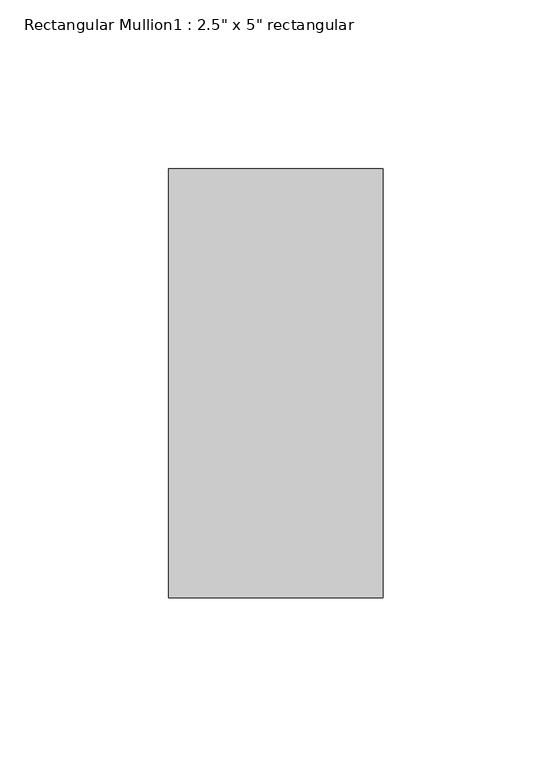
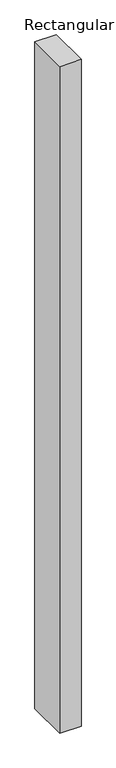
"""IFC4 building model written with IfcOpenShell, lengths in millimetres: member geometry."""

import ifcopenshell
import ifcopenshell.guid

model = None  # the IFC model being written
_history = None  # IfcOwnerHistory: only IFC2X3 demands one
_inside = {}  # id of a spatial element -> (the spatial element, [elements in it])
_under = {}  # id of a project, library or spatial element -> (it, [spatial elements below it])
_declared = {}  # id of a project -> (the project, [libraries it declares])
_typed = {}  # id of a type object -> (the type object, [elements of that type])
_made_of = {}  # id of a material, layer set ... -> (it, [elements and type objects made of it])


def new_model(schema):
    """Start an empty IFC model of exactly this schema.

    Asked for "IFC4X3", IfcOpenShell would pick the latest addendum, in which some entities
    have other attributes; the version numbers below select the first issue.
    IFC2X3 requires an IfcOwnerHistory on every rooted entity: one is made here for all.
    """
    global model, _history
    if schema == "IFC4X3":
        model = ifcopenshell.file(schema_version=(4, 3, 0, 0))
    else:
        model = ifcopenshell.file(schema=schema)
    _inside.clear()
    _under.clear()
    _declared.clear()
    _typed.clear()
    _made_of.clear()
    _history = None
    if model.schema == "IFC2X3":
        org = make("IfcOrganization", Name="unknown")
        user = make(
            "IfcPersonAndOrganization",
            ThePerson=make("IfcPerson", FamilyName="unknown"),
            TheOrganization=org,
        )
        app = make(
            "IfcApplication",
            ApplicationDeveloper=org,
            Version="unknown",
            ApplicationFullName="unknown",
            ApplicationIdentifier="unknown",
        )
        _history = make(
            "IfcOwnerHistory",
            OwningUser=user,
            OwningApplication=app,
            ChangeAction="ADDED",
            CreationDate=0,
        )
    return model


def make(cls, **values):
    """One entity of the class cls with the attributes given. An attribute that is None is left unset."""
    return model.create_entity(
        cls, **{name: value for name, value in values.items() if value is not None}
    )


def rooted(cls, **values):
    """An entity with a GlobalId (a new one), such as an element, a storey or a relation."""
    return make(cls, GlobalId=ifcopenshell.guid.new(), OwnerHistory=_history, **values)


def si_unit(unit_type, name, prefix=None):
    """IfcSIUnit, for example si_unit("LENGTHUNIT", "METRE", prefix="MILLI")."""
    return make("IfcSIUnit", UnitType=unit_type, Prefix=prefix, Name=name)


def assignment(units):
    """IfcUnitAssignment: the units of a project."""
    return None if units is None else make("IfcUnitAssignment", Units=units)


def point(xyz):
    """IfcCartesianPoint."""
    return None if xyz is None else make("IfcCartesianPoint", Coordinates=xyz)


def direction(xyz):
    """IfcDirection."""
    return None if xyz is None else make("IfcDirection", DirectionRatios=xyz)


def frame(location, z_axis=None, x_axis=None):
    """IfcAxis2Placement3D, a coordinate frame: its origin and axes. An axis left out is left unset."""
    return make(
        "IfcAxis2Placement3D",
        Location=point(location),
        Axis=direction(z_axis),
        RefDirection=direction(x_axis),
    )


def origin():
    """The frame at (0, 0, 0) with its axes left unset."""
    return frame((0.0, 0.0, 0.0))


def place(relative_to, where):
    """IfcLocalPlacement: puts the frame where relative to a parent placement (None: the world)."""
    return make(
        "IfcLocalPlacement", PlacementRelTo=relative_to, RelativePlacement=where
    )


def context(
    kind, dimensions, precision=None, world=None, true_north=None, identifier=None
):
    """IfcGeometricRepresentationContext, for example the 3D "Model" context."""
    return make(
        "IfcGeometricRepresentationContext",
        ContextIdentifier=identifier,
        ContextType=kind,
        CoordinateSpaceDimension=dimensions,
        Precision=precision,
        WorldCoordinateSystem=world,
        TrueNorth=true_north,
    )


def project(units=None, contexts=None):
    """IfcProject with its units and contexts."""
    return rooted(
        "IfcProject",
        Name="project",
        RepresentationContexts=contexts,
        UnitsInContext=assignment(units),
    )


def spatial(cls, under=None, at=None, **own):
    """A site, building, storey or space (cls), placed at a placement, below another one or the project."""
    s = rooted(cls, ObjectPlacement=at, **own)
    if under is not None:
        _under.setdefault(under.id(), (under, []))[1].append(s)
    return s


def polyline(points):
    """IfcPolyline through the points."""
    return make("IfcPolyline", Points=[point(p) for p in points])


def outline(outer, holes=None, kind="AREA"):
    """IfcArbitraryClosedProfileDef: a profile drawn as a closed curve; with holes, ...WithVoids."""
    if holes is None:
        return make("IfcArbitraryClosedProfileDef", ProfileType=kind, OuterCurve=outer)
    return make(
        "IfcArbitraryProfileDefWithVoids",
        ProfileType=kind,
        OuterCurve=outer,
        InnerCurves=holes,
    )


def extrude(swept, where, along, depth):
    """IfcExtrudedAreaSolid: the profile swept, set in the frame where, extruded along a direction by depth."""
    return make(
        "IfcExtrudedAreaSolid",
        SweptArea=swept,
        Position=where,
        ExtrudedDirection=direction(along),
        Depth=depth,
    )


def shape(context_of_items, identifier, shape_type, items):
    """IfcShapeRepresentation: the items that make up one representation, for example the "Body"."""
    return make(
        "IfcShapeRepresentation",
        ContextOfItems=context_of_items,
        RepresentationIdentifier=identifier,
        RepresentationType=shape_type,
        Items=items,
    )


def source(mapping_origin, context_of_items, identifier, shape_type, items):
    """IfcRepresentationMap: a shape defined once, which mapped items show again and again."""
    return make(
        "IfcRepresentationMap",
        MappingOrigin=mapping_origin,
        MappedRepresentation=shape(context_of_items, identifier, shape_type, items),
    )


def transform(
    local_origin,
    x_axis=None,
    y_axis=None,
    z_axis=None,
    scale=None,
    scale2=None,
    scale3=None,
    uniform=True,
):
    """IfcCartesianTransformationOperator3D, or its non-uniform kind. x_axis, y_axis, z_axis: its Axis1, 2, 3."""
    if uniform:
        return make(
            "IfcCartesianTransformationOperator3D",
            Axis1=direction(x_axis),
            Axis2=direction(y_axis),
            LocalOrigin=point(local_origin),
            Scale=scale,
            Axis3=direction(z_axis),
        )
    return make(
        "IfcCartesianTransformationOperator3DnonUniform",
        Axis1=direction(x_axis),
        Axis2=direction(y_axis),
        LocalOrigin=point(local_origin),
        Scale=scale,
        Axis3=direction(z_axis),
        Scale2=scale2,
        Scale3=scale3,
    )


def mapped(mapping_source, mapping_target):
    """IfcMappedItem: shows the shape of a source again, moved by a transform."""
    return make(
        "IfcMappedItem", MappingSource=mapping_source, MappingTarget=mapping_target
    )


def made_of(thing, what):
    """Note that an element or type object is made of a material, layer set ...; save() writes the relation."""
    if what is not None:
        _made_of.setdefault(what.id(), (what, []))[1].append(thing)
    return thing


def element(
    cls,
    number,
    at=None,
    inside=None,
    cuts=None,
    type_object=None,
    material=None,
    context=None,
    identifier="Body",
    shape_type=None,
    held_by="IfcProductDefinitionShape",
    body=None,
    shapes=None,
    **own,
):
    """One element of the class cls, such as IfcWall. Its Tag is "e" and its number.

    at: its placement. inside: the storey or other place that contains it. cuts: it is an
    opening in that element (IfcRelVoidsElement). A single representation is given by context,
    identifier, shape_type and body (its items); several are given by shapes. held_by: the class
    of the entity that holds the representations. save() writes the other relations.
    """
    e = rooted(cls, Tag="e%d" % number, ObjectPlacement=at, **own)
    if body is not None:
        shapes = [shape(context, identifier, shape_type, body)]
    if shapes is not None:
        e.Representation = make(held_by, Representations=shapes)
    if inside is not None:
        _inside.setdefault(inside.id(), (inside, []))[1].append(e)
    if cuts is not None:
        rooted(
            "IfcRelVoidsElement", RelatingBuildingElement=cuts, RelatedOpeningElement=e
        )
    if type_object is not None:
        _typed.setdefault(type_object.id(), (type_object, []))[1].append(e)
    return made_of(e, material)


def aggregate(whole, parts):
    """IfcRelAggregates: a whole, such as a stair, and the parts it consists of."""
    return rooted("IfcRelAggregates", RelatingObject=whole, RelatedObjects=parts)


def save(model, path):
    """Write the relations noted so far, then the file.

    IfcRelAggregates (storeys below a building ...), IfcRelContainedInSpatialStructure (elements
    in a storey), IfcRelDefinesByType, IfcRelAssociatesMaterial and IfcRelDeclares: one each for
    every whole, place, type object, material and project.
    """
    for whole, parts in _under.values():
        aggregate(whole, parts)
    for where, things in _inside.values():
        rooted(
            "IfcRelContainedInSpatialStructure",
            RelatedElements=things,
            RelatingStructure=where,
        )
    for kind, things in _typed.values():
        rooted("IfcRelDefinesByType", RelatedObjects=things, RelatingType=kind)
    for what, things in _made_of.values():
        rooted("IfcRelAssociatesMaterial", RelatedObjects=things, RelatingMaterial=what)
    for by, libraries in _declared.values():
        rooted("IfcRelDeclares", RelatingContext=by, RelatedDefinitions=libraries)
    model.write(path)


def member_a397286f(model_context):
    return source(origin(), model_context, "Body", "SweptSolid", [
        extrude(outline(polyline([(0.0, 63.5), (0.0, -63.5), (-63.5, -63.5), (-63.5, 63.5), (0.0, 63.5)])), frame((0.0, 0.0, -2091.69), z_axis=(0.0, 0.0, 1.0), x_axis=(1.0, 0.0, 0.0)), (0.0, 0.0, 1.0), 2091.69),
    ])


if __name__ == "__main__":
    model = new_model("IFC4")
    model_context = context("Model", 3, world=origin())
    ifc_project = project(units=[si_unit("LENGTHUNIT", "METRE", prefix="MILLI")], contexts=[model_context])
    site = spatial("IfcSite", under=ifc_project)
    building = spatial("IfcBuilding", under=site)
    placement = place(None, origin())
    member_shape = member_a397286f(model_context)
    element("IfcMember", 1, ObjectType="Rectangular Mullion1 : 2.5\" x 5\" rectangular", at=placement, inside=building, context=model_context, shape_type="MappedRepresentation", body=[
        mapped(member_shape, transform((0.0, 0.0, 0.0), x_axis=(1.0, 0.0, 0.0), y_axis=(0.0, 1.0, 0.0), z_axis=(0.0, 0.0, 1.0))),
    ])
    save(model, "model.ifc")

# Revit data of these elements
# Type "Rectangular Mullion1 : 2.5\" x 5\" rectangular"
#   built-in parameter 1007304 = 0.416667 (stored number, unit not read)
#   built-in parameter 1007301 = 0.104167 (stored number, unit not read)
#   built-in parameter 1007300 = 0.104167 (stored number, unit not read)
# Element 1 (IfcMember, "Rectangular Mullion1 : 2.5\" x 5\" rectangular")
#   Materials on its faces: "support-frame"
# Materials
#   "support-frame": class "Unassigned", colour RGB 233 233 233, transparency 0, Cost = 0
